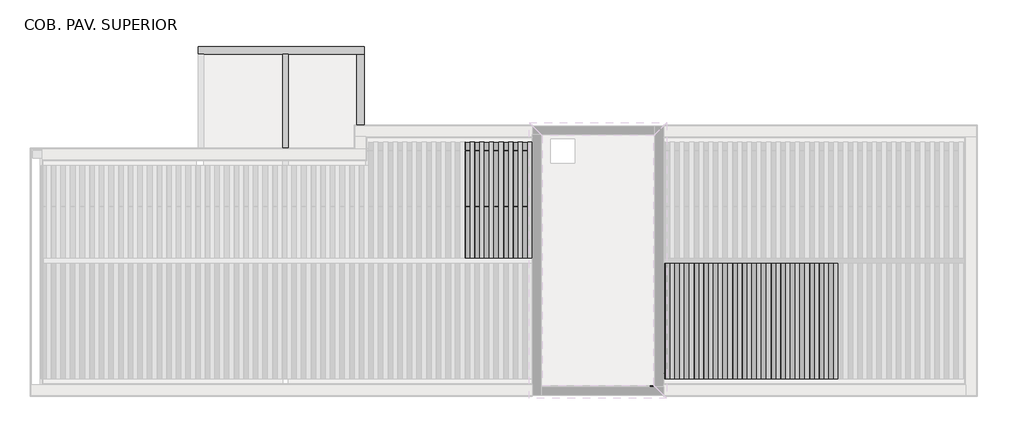
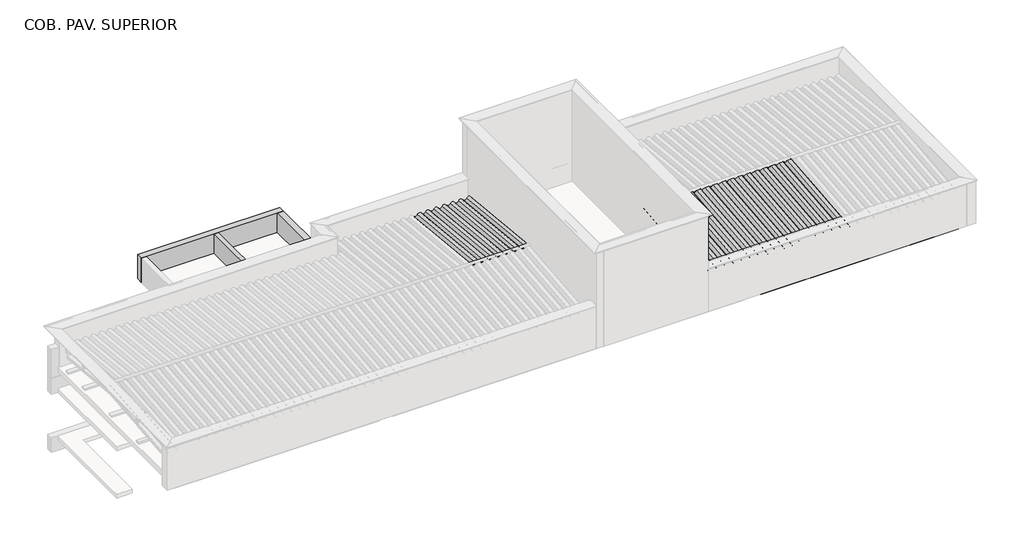
# One storey, part 5 of 7: 41 beams, 9 columns.
# Revit data of these elements (continued)
# Type "Madeira de lei : Berço 6x12cm"
#   A = 0.02 m²
#   Length [instance default] = 1.524 m
#   b = 0.06 m
#   d = 0.12 m
#   Structural Material [instance default] = none
#   Assembly Code = ""
# Type "TQS - Viga retangular : 14.0 x 76.0"
#   Length [instance default] = 1.524 m
#   b = 0.14 m
#   h = 0.76 m
#   Structural Material [instance default] = none
#   Assembly Code = ""
# Type "TQS - Viga retangular : 19.0 x 60.0"
#   Length [instance default] = 1.524 m
#   b = 0.19 m
#   h = 0.60 m
#   Structural Material [instance default] = none
#   Assembly Code = ""
# Type "TQS - Viga retangular : 19.0 x 76.0"
#   Length [instance default] = 1.524 m
#   b = 0.19 m
#   h = 0.76 m
#   Structural Material [instance default] = none
#   Assembly Code = ""
# Type "TQS - Viga retangular : 19.0 x 80.0"
#   Length [instance default] = 1.524 m
#   b = 0.19 m
#   h = 0.80 m
#   Structural Material [instance default] = none
#   Assembly Code = ""
# Type "Telha Ondulada : Fibrocimento"
#   Description = "TELHA ONDULADA FIBROCIMENTO"
#   Cost = 5
#   Length [instance default] = 1.524 m
#   b = 0.07 m
#   h = 0.16 m
#   Structural Material = .TELHA DE FIBROCIMENTO
#   Assembly Code = ""
# Type "Madeira de lei-Coluna : Pontalete 6X16cm"
#   A = 0.01952 m²
#   b = 0.06 m
#   d = 0.16 m
#   Structural Material [instance default] = none
#   Assembly Code = ""
# Type "TQS - Pilar retangular : 19.0 x 30.0"
#   b = 0.19 m
#   h = 0.30 m
#   Structural Material [instance default] = Concrete - Cast-in-Place Concrete
# Elements 1, 2, 3, 4, 5, 6, 7, 8, 9, 10 (IfcBeam, "Madeira de lei : Berço 6x12cm")
#   Comments = ""
#   Structural Material = .MADEIRAMENTO
#   Phase Created = CC_PE
#   Materials on its faces: ".MADEIRAMENTO"
# Element 11 (IfcBeam, "TQS - Viga retangular : 14.0 x 76.0")
#   Uso = "ESTRUTURA"
#   Titulo = "V417"
#   Chave = "-401"
#   Tipo Elemento = "Viga"
#   SHA1 = "EC21F3857AF6ADE151F31ED353C555F6460C2153"
#   Revisão = ""
#   Tipo de carga = ""
#   Divisor de flexao = ""
#   Secao = ""
#   Configuracao = ""
#   Angulo (graus) = ""
#   Detalhamento = ""
#   Casos de vento manual = ""
#   Tipo = ""
#   Alcas = ""
#   Furos = ""
#   Pino = ""
#   Distribuicao = ""
#   Solidarizado = ""
#   Solidarizar na montagem = ""
#   Unir com o próximo = ""
#   Grupo pre moldado = ""
#   Verificado = ""
#   Concreto C = ""
#   Taxa de armadura (kgf/m³) = 0
#   Carga (tf/m²) = 0
#   Carga (tf/m) = 0
#   Carga (tf) = 0
#   Altura = 0.76 m
#   Rebaixo = -0.40 m
#   Largura = 0.14 m
#   Distancia a face = 0.00 m
#   Distancia ao eixo = 0.00 m
#   Altura gerber esquerda = 0.00 m
#   Largura gerber esquerda = 0.00 m
#   Altura gerber direita = 0.00 m
#   Largura gerber direita = 0.00 m
#   Resultado de Ensaios fck (MPa) = 0
#   Unique TQS ID = -401
#   Principal = yes
#   Structural Material = none
#   Phase Created = CC_PE
# Element 12 (IfcBeam, "TQS - Viga retangular : 19.0 x 60.0")
#   Uso = "ESTRUTURA"
#   Titulo = "V419"
#   Chave = "-1306"
#   Tipo Elemento = "Viga"
#   SHA1 = "D71F304D6FDB9A66A15A372791015F707934082B"
#   Revisão = ""
#   Tipo de carga = ""
#   Divisor de flexao = ""
#   Secao = ""
#   Configuracao = ""
#   Angulo (graus) = ""
#   Detalhamento = ""
#   Casos de vento manual = ""
#   Tipo = ""
#   Alcas = ""
#   Furos = ""
#   Pino = ""
#   Distribuicao = ""
#   Solidarizado = ""
#   Solidarizar na montagem = ""
#   Unir com o próximo = ""
#   Grupo pre moldado = ""
#   Verificado = ""
#   Concreto C = ""
#   Taxa de armadura (kgf/m³) = 0
#   Carga (tf/m²) = 0
#   Carga (tf/m) = 0
#   Carga (tf) = 0
#   Altura = 0.60 m
#   Rebaixo = -0.40 m
#   Largura = 0.19 m
#   Distancia a face = 0.00 m
#   Distancia ao eixo = 0.00 m
#   Altura gerber esquerda = 0.00 m
#   Largura gerber esquerda = 0.00 m
#   Altura gerber direita = 0.00 m
#   Largura gerber direita = 0.00 m
#   Resultado de Ensaios fck (MPa) = 0
#   Unique TQS ID = -1306
#   Principal = yes
#   Structural Material = none
#   Phase Created = CC_PE
# Element 13 (IfcBeam, "TQS - Viga retangular : 19.0 x 76.0")
#   Uso = "ESTRUTURA"
#   Titulo = "V401"
#   Chave = "-409"
#   Tipo Elemento = "Viga"
#   SHA1 = "F7B43E387DF096475B2F8EBA1B47A3499C7AD8F9"
#   Revisão = ""
#   Tipo de carga = ""
#   Divisor de flexao = ""
#   Secao = ""
#   Configuracao = ""
#   Angulo (graus) = ""
#   Detalhamento = ""
#   Casos de vento manual = ""
#   Tipo = ""
#   Alcas = ""
#   Furos = ""
#   Pino = ""
#   Distribuicao = ""
#   Solidarizado = ""
#   Solidarizar na montagem = ""
#   Unir com o próximo = ""
#   Grupo pre moldado = ""
#   Verificado = ""
#   Concreto C = ""
#   Taxa de armadura (kgf/m³) = 0
#   Carga (tf/m²) = 0
#   Carga (tf/m) = 0
#   Carga (tf) = 0
#   Altura = 0.76 m
#   Rebaixo = -0.40 m
#   Largura = 0.19 m
#   Distancia a face = 0.00 m
#   Distancia ao eixo = 0.00 m
#   Altura gerber esquerda = 0.00 m
#   Largura gerber esquerda = 0.00 m
#   Altura gerber direita = 0.00 m
#   Largura gerber direita = 0.00 m
#   Resultado de Ensaios fck (MPa) = 0
#   Unique TQS ID = -409
#   Principal = yes
#   Structural Material = none
#   Phase Created = CC_PE
# Element 14 (IfcBeam, "TQS - Viga retangular : 19.0 x 76.0")
#   Uso = "ESTRUTURA"
#   Titulo = "V418"
#   Chave = "-506"
#   Tipo Elemento = "Viga"
#   SHA1 = "CDFDF13DA9DFF6C4F16A197A7E285328A49A230D"
#   Revisão = ""
#   Tipo de carga = ""
#   Divisor de flexao = ""
#   Secao = ""
#   Configuracao = ""
#   Angulo (graus) = ""
#   Detalhamento = ""
#   Casos de vento manual = ""
#   Tipo = ""
#   Alcas = ""
#   Furos = ""
#   Pino = ""
#   Distribuicao = ""
#   Solidarizado = ""
#   Solidarizar na montagem = ""
#   Unir com o próximo = ""
#   Grupo pre moldado = ""
#   Verificado = ""
#   Concreto C = ""
#   Taxa de armadura (kgf/m³) = 0
#   Carga (tf/m²) = 0
#   Carga (tf/m) = 0
#   Carga (tf) = 0
#   Altura = 0.76 m
#   Rebaixo = -0.40 m
#   Largura = 0.19 m
#   Distancia a face = 0.00 m
#   Distancia ao eixo = 0.00 m
#   Altura gerber esquerda = 0.00 m
#   Largura gerber esquerda = 0.00 m
#   Altura gerber direita = 0.00 m
#   Largura gerber direita = 0.00 m
#   Resultado de Ensaios fck (MPa) = 0
#   Unique TQS ID = -506
#   Principal = yes
#   Structural Material = none
#   Phase Created = CC_PE
# Element 15 (IfcBeam, "TQS - Viga retangular : 19.0 x 80.0")
#   Uso = "ESTRUTURA"
#   Titulo = "V411"
#   Chave = "-395"
#   Tipo Elemento = "Viga"
#   SHA1 = "58756CC417DAC53D595605301D556BE3FCA3E4A2"
#   Revisão = ""
#   Tipo de carga = ""
#   Divisor de flexao = ""
#   Secao = ""
#   Configuracao = ""
#   Angulo (graus) = ""
#   Detalhamento = ""
#   Casos de vento manual = ""
#   Tipo = ""
#   Alcas = ""
#   Furos = ""
#   Pino = ""
#   Distribuicao = ""
#   Solidarizado = ""
#   Solidarizar na montagem = ""
#   Unir com o próximo = ""
#   Grupo pre moldado = ""
#   Verificado = ""
#   Concreto C = ""
#   Taxa de armadura (kgf/m³) = 0
#   Carga (tf/m²) = 0
#   Carga (tf/m) = 0
#   Carga (tf) = 0
#   Altura = 0.80 m
#   Rebaixo = -0.60 m
#   Largura = 0.19 m
#   Distancia a face = 0.00 m
#   Distancia ao eixo = 0.00 m
#   Altura gerber esquerda = 0.00 m
#   Largura gerber esquerda = 0.00 m
#   Altura gerber direita = 0.00 m
#   Largura gerber direita = 0.00 m
#   Resultado de Ensaios fck (MPa) = 0
#   Unique TQS ID = -395
#   Principal = yes
#   Structural Material = none
#   Phase Created = CC_PE
# Element 16 (IfcBeam, "TQS - Viga retangular : 19.0 x 80.0")
#   Uso = "ESTRUTURA"
#   Titulo = "V402"
#   Chave = "-498"
#   Tipo Elemento = "Viga"
#   SHA1 = "7F1FF78245035ACB38743B8022C1D89C5ED7777C"
#   Revisão = ""
#   Tipo de carga = ""
#   Divisor de flexao = ""
#   Secao = ""
#   Configuracao = ""
#   Angulo (graus) = ""
#   Detalhamento = ""
#   Casos de vento manual = ""
#   Tipo = ""
#   Alcas = ""
#   Furos = ""
#   Pino = ""
#   Distribuicao = ""
#   Solidarizado = ""
#   Solidarizar na montagem = ""
#   Unir com o próximo = ""
#   Grupo pre moldado = ""
#   Verificado = ""
#   Concreto C = ""
#   Taxa de armadura (kgf/m³) = 0
#   Carga (tf/m²) = 0
#   Carga (tf/m) = 0
#   Carga (tf) = 0
#   Altura = 0.80 m
#   Rebaixo = -0.60 m
#   Largura = 0.19 m
#   Distancia a face = 0.00 m
#   Distancia ao eixo = 0.00 m
#   Altura gerber esquerda = 0.00 m
#   Largura gerber esquerda = 0.00 m
#   Altura gerber direita = 0.00 m
#   Largura gerber direita = 0.00 m
#   Resultado de Ensaios fck (MPa) = 0
#   Unique TQS ID = -498
#   Principal = yes
#   Structural Material = none
#   Phase Created = CC_PE
# Elements 17, 18, 19, 20, 21, 22, 23, 24, 25, 26, 27, 28, 29, 30, 31, 32, 33, 34, 35, 36, 37, 38, 39, 40, 41 (IfcBeam, "Telha Ondulada : Fibrocimento")
#   Phase Created = CC_PE
#   Materials on its faces: ".TELHA DE FIBROCIMENTO"
# Elements 42, 43, 44, 45, 46, 47, 48, 49 (IfcColumn, "Madeira de lei-Coluna : Pontalete 6X16cm")
#   Comments = ""
#   Structural Material = .MADEIRAMENTO
#   Phase Created = CC_PE
#   Materials on its faces: ".MADEIRAMENTO"
# Element 50 (IfcColumn, "TQS - Pilar retangular : 19.0 x 30.0")
#   Uso = "ESTRUTURA"
#   Titulo = "PT2"
#   Chave = "PT2//0"
#   Tipo Elemento = "Pilar"
#   SHA1 = "F43D605D1DA00D757641A848CE7023BEF37C9FDC"
#   Revisão = ""
#   Tipo de carga = ""
#   Divisor de flexao = ""
#   Secao = "R 19/30 90°"
#   Configuracao = ""
#   Angulo (graus) = ""
#   Detalhamento = ""
#   Casos de vento manual = ""
#   Tipo = ""
#   Alcas = ""
#   Furos = ""
#   Pino = ""
#   Distribuicao = ""
#   Solidarizado = ""
#   Solidarizar na montagem = ""
#   Unir com o próximo = ""
#   Grupo pre moldado = ""
#   Verificado = ""
#   Concreto C = ""
#   Taxa de armadura (kgf/m³) = 0
#   Carga (tf/m²) = 0
#   Carga (tf/m) = 0
#   Carga (tf) = 0
#   Altura = 2.10 m
#   Rebaixo = 0.00 m
#   Altura da fundacao = 0.00 m
#   Largura = 0.00 m
#   Distancia a face = 0.00 m
#   Distancia ao eixo = 0.00 m
#   Resultado de Ensaios fck (MPa) = 0
#   Unique TQS ID = -428
#   Principal = yes
#   Nasce = yes
#   Morre = yes
#   Cabeca de Pilar = no
#   Structural Material = Concrete - Cast-in-Place Concrete
#   Phase Created = CC_PE
#   Materials on its faces: "Concrete - Cast-in-Place Concrete"
# Materials
#   ".TELHA DE FIBROCIMENTO": class "CC_TELHADO", colour RGB 77 77 76, transparency 0, Description = "TELHA ONDULADA FIBROCIMENTO", Cost = 0
#   "Concrete - Cast-in-Place Concrete": class "Unassigned", colour RGB 192 192 192, transparency 0
#   ".MADEIRAMENTO": class ".CC_MADEIRAS", colour RGB 212 179 113, transparency 0, Cost = 0
